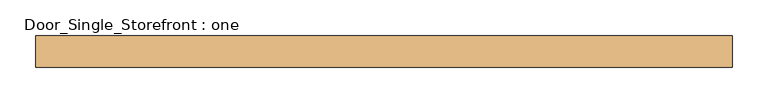
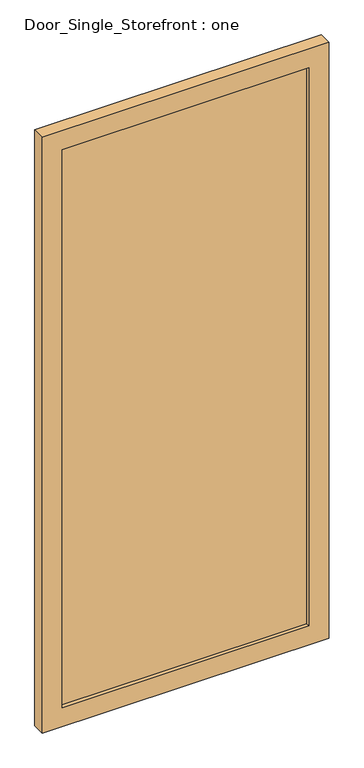
"""IFC4 building model written with IfcOpenShell, lengths in millimetres: door geometry, Door_Single_Storefront : one."""

from ifc_helpers import new_model, si_unit, frame, origin, place, context, project, spatial, polyline, outline, extrude, source, transform, mapped, element, save


def door_single_storefront_one_19de2b64(model_context):
    return source(origin(), model_context, "Body", "SweptSolid", [
        extrude(outline(polyline([(421.878125, -6.35), (-421.878125, -6.35), (-421.878125, 12.7), (421.878125, 12.7), (421.878125, -6.35)])), frame((0.0, 0.0, 68.2625), z_axis=(0.0, 0.0, 1.0), x_axis=(1.0, 0.0, 0.0)), (0.0, 0.0, 1.0), 2016.125),
        extrude(outline(polyline([(2152.65, -490.140625), (0.0, -490.140625), (0.0, 490.140625), (2152.65, 490.140625), (2152.65, -490.140625)]), holes=[polyline([(68.2625, 421.878125), (68.2625, -421.878125), (2084.3875, -421.878125), (2084.3875, 421.878125), (68.2625, 421.878125)])]), frame((0.0, -19.05, 0.0), z_axis=(0.0, 1.0, 0.0), x_axis=(0.0, 0.0, 1.0)), (0.0, 0.0, 1.0), 44.45),
    ])


if __name__ == "__main__":
    model = new_model("IFC4")
    model_context = context("Model", 3, world=origin())
    ifc_project = project(units=[si_unit("LENGTHUNIT", "METRE", prefix="MILLI")], contexts=[model_context])
    site = spatial("IfcSite", under=ifc_project)
    building = spatial("IfcBuilding", under=site)
    placement = place(None, origin())
    door_single_storefront_one_shape = door_single_storefront_one_19de2b64(model_context)
    element("IfcDoor", 1, ObjectType="Door_Single_Storefront : one", at=placement, inside=building, context=model_context, shape_type="MappedRepresentation", body=[
        mapped(door_single_storefront_one_shape, transform((0.0, 0.0, 0.0), x_axis=(1.0, 0.0, 0.0), y_axis=(0.0, 1.0, 0.0), z_axis=(0.0, 0.0, 1.0))),
    ])
    save(model, "model.ifc")

# Revit data of these elements
# Type "Door_Single_Storefront : one"
#   Type Mark = "29"
#   OD_DS_Door_Material = "ALUM./GLAZING"
#   OD_DS_Door_Type = "STOREFRONT (NARROW STILE)"
#   OD_DS_Lockset = "ENTRY LOCK (INSIDE ADA LEVER ALWAYS ACTIVE)"
#   Analytic Construction = "<None>"
#   angle open [instance default] = 132.952°
#   Stile_Width = 0' - 2 11/16"
#   Door_Thickness = 0' - 1 3/4"
#   Door_Offset = 0' - 1"
#   Glass_Material = TEMPERED INSULATED GLAZING (CARDINAL GLASS LoĒ²-240\nOR EQUIVALENT)
#   Frame_Material = KAWNEER 260 INSULCLADTM THERMAL ENTRANCE - CLEAR ANODIZED ALUM.
#   Function = (empty or 0)
# Element 1 (IfcDoor, "Door_Single_Storefront : one")
#   angle open = 170.00°
#   Materials on its faces: "KAWNEER 260 INSULCLADTM THERMAL ENTRANCE - CLEAR ANODIZED ALUM.", "TEMPERED INSULATED GLAZING (CARDINAL GLASS LoĒ²-240\nOR EQUIVALENT)"
# Materials
#   "TEMPERED INSULATED GLAZING (CARDINAL GLASS LoĒ²-240\nOR EQUIVALENT)": class "Glass", colour RGB 196 205 210, transparency 0.85, Description = "Soda Lime Glass", Cost = 0
#   "KAWNEER 260 INSULCLADTM THERMAL ENTRANCE - CLEAR ANODIZED ALUM.": class "Metal", colour RGB 244 244 244, transparency 0, Description = "Aluminum 6061", Cost = 0
